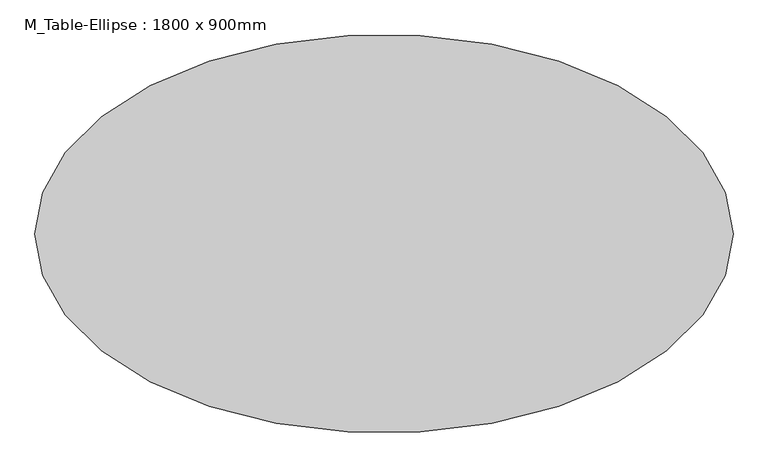
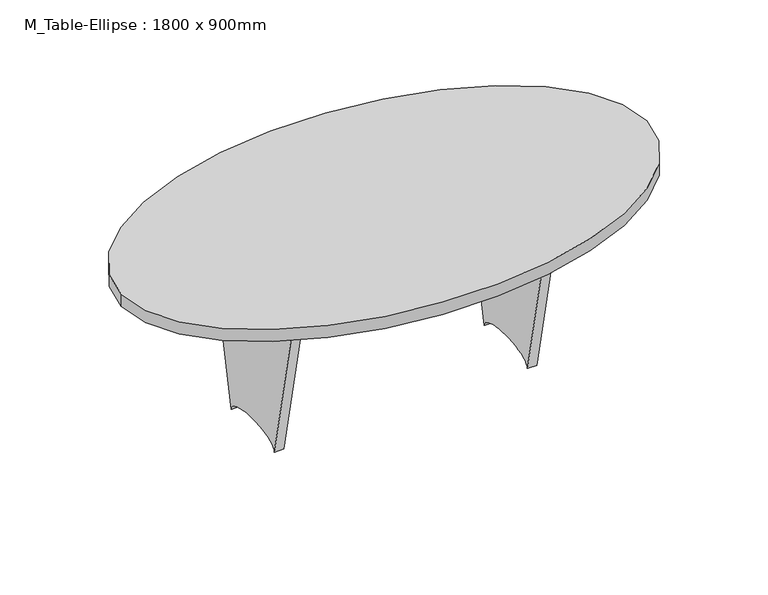
"""IFC4 building model written with IfcOpenShell, lengths in millimetres: furniture geometry, M_Table-Ellipse : 1800 x 900mm."""

from ifc_helpers import new_model, si_unit, point, frame, origin, place, context, project, spatial, ellipse_curve, trimmed, source, transform, mapped, element, save
from ifc_brep_helpers import plane_surface, extruded_surface, advanced_brep


def m_table_ellipse_1800_x_900mm_170b96be(model_context):
    return source(origin(), model_context, "Body", "AdvancedBrep", [
        advanced_brep(
        [(-486.9, 19.05, 709.2), (486.9, 19.05, 709.2), (486.9, 19.05, 472.8), (-486.9, 19.05, 472.8), (-486.9, -19.05, 709.2), (-486.9, -19.05, 472.8), (486.9, -19.05, 472.8), (486.9, -19.05, 709.2)],
        [
            (0, 1),
            (1, 2),
            (2, 3, ellipse_curve(frame((0.0, 19.05, 472.8), z_axis=(0.0, -1.0, 0.0), x_axis=(1.0, 0.0, 0.0)), 486.9, 101.6)),
            (3, 0),
            (4, 5),
            (5, 6, ellipse_curve(frame((0.0, -19.05, 472.8), z_axis=(0.0, 1.0, 0.0), x_axis=(1.0, 0.0, 0.0)), 486.9, 101.6)),
            (6, 7),
            (7, 4),
            (0, 4),
            (7, 1),
            (6, 2),
            (5, 3),
        ],
        [
            plane_surface(frame((-486.9, 19.05, 709.2), z_axis=(0.0, 1.0, 0.0), x_axis=(1.0, 0.0, 0.0))),
            plane_surface(frame((-486.9, -19.05, 709.2), z_axis=(0.0, -1.0, 0.0), x_axis=(-1.0, 0.0, 0.0))),
            plane_surface(frame((-486.9, 19.05, 709.2), z_axis=(0.0, 0.0, 1.0), x_axis=(0.0, -1.0, 0.0))),
            plane_surface(frame((486.9, 19.05, 709.2), z_axis=(1.0, 0.0, 0.0), x_axis=(0.0, -1.0, 0.0))),
            extruded_surface(trimmed(ellipse_curve(frame((0.0, -57.15, 472.8), z_axis=(0.0, -1.0, 0.0), x_axis=(1.0, 0.0, 0.0)), 486.9, 101.6), [point((486.9, -57.15, 472.8))], [point((-486.9, -57.15, 472.8))], True, "CARTESIAN"), (0.0, 38.099999999999994, 0.0), 38.099999999999994),
            plane_surface(frame((-486.9, 19.05, 472.8), z_axis=(-1.0, 0.0, 0.0), x_axis=(0.0, -1.0, 0.0))),
        ],
        [
            (0, [[1, 2, 3, 4]]),
            (1, [[5, 6, 7, 8]]),
            (2, [[-1, 9, -8, 10]]),
            (3, [[-2, -10, -7, 11]]),
            (4, [[-3, -11, -6, 12]]),
            (5, [[-4, -12, -5, -9]]),
        ],
    ),
        advanced_brep(
        [(525.0, 300.0, 709.2), (525.0, -300.0, 709.2), (525.0, -150.0, 0.0), (525.0, 150.0, 0.0), (486.9, 300.0, 709.2), (486.9, 150.0, 0.0), (486.9, -150.0, 0.0), (486.9, -300.0, 709.2)],
        [
            (0, 1),
            (1, 2),
            (2, 3, ellipse_curve(frame((525.0, 0.0, 0.0), z_axis=(-1.0, 0.0, 0.0), x_axis=(0.0, 1.0, 0.0)), 150.0, 50.8)),
            (3, 0),
            (4, 5),
            (5, 6, ellipse_curve(frame((486.9, 0.0, 0.0), z_axis=(1.0, 0.0, 0.0), x_axis=(0.0, 1.0, 0.0)), 150.0, 50.8)),
            (6, 7),
            (7, 4),
            (0, 4),
            (7, 1),
            (6, 2),
            (5, 3),
        ],
        [
            plane_surface(frame((525.0, -300.0, 709.2), z_axis=(1.0, 0.0, 0.0), x_axis=(0.0, -1.0, 0.0))),
            plane_surface(frame((486.9, -300.0, 709.2), z_axis=(-1.0, 0.0, 0.0), x_axis=(0.0, 1.0, 0.0))),
            plane_surface(frame((525.0, 300.0, 709.2), z_axis=(0.0, 0.0, 1.0), x_axis=(-1.0, 0.0, 0.0))),
            plane_surface(frame((525.0, -300.0, 709.2), z_axis=(0.0, -0.9783561485468907, -0.206928119405011), x_axis=(-1.0, 0.0, 0.0))),
            extruded_surface(trimmed(ellipse_curve(frame((448.8, 0.0, 0.0), z_axis=(-1.0, 0.0, 0.0), x_axis=(0.0, 1.0, 0.0)), 150.0, 50.8), [point((448.8, -150.0, 0.0))], [point((448.8, 150.0, 0.0))], True, "CARTESIAN"), (38.099999999999966, 0.0, 0.0), 38.099999999999966),
            plane_surface(frame((525.0, 150.0, 0.0), z_axis=(0.0, 0.9783561485468916, -0.2069281194050069), x_axis=(-1.0, 0.0, 0.0))),
        ],
        [
            (0, [[1, 2, 3, 4]]),
            (1, [[5, 6, 7, 8]]),
            (2, [[-1, 9, -8, 10]]),
            (3, [[-2, -10, -7, 11]]),
            (4, [[-3, -11, -6, 12]]),
            (5, [[-4, -12, -5, -9]]),
        ],
    ),
        advanced_brep(
        [(-486.9, 300.0, 709.2), (-486.9, -300.0, 709.2), (-486.9, -150.0, 0.0), (-486.9, 150.0, 0.0), (-525.0, 300.0, 709.2), (-525.0, 150.0, 0.0), (-525.0, -150.0, 0.0), (-525.0, -300.0, 709.2)],
        [
            (0, 1),
            (1, 2),
            (2, 3, ellipse_curve(frame((-486.9, 0.0, 0.0), z_axis=(-1.0, 0.0, 0.0), x_axis=(0.0, 1.0, 0.0)), 150.0, 50.8)),
            (3, 0),
            (4, 5),
            (5, 6, ellipse_curve(frame((-525.0, 0.0, 0.0), z_axis=(1.0, 0.0, 0.0), x_axis=(0.0, 1.0, 0.0)), 150.0, 50.8)),
            (6, 7),
            (7, 4),
            (0, 4),
            (7, 1),
            (6, 2),
            (5, 3),
        ],
        [
            plane_surface(frame((-486.9, -300.0, 709.2), z_axis=(1.0, 0.0, 0.0), x_axis=(0.0, -1.0, 0.0))),
            plane_surface(frame((-525.0, -300.0, 709.2), z_axis=(-1.0, 0.0, 0.0), x_axis=(0.0, 1.0, 0.0))),
            plane_surface(frame((-486.9, 300.0, 709.2), z_axis=(0.0, 0.0, 1.0), x_axis=(-1.0, 0.0, 0.0))),
            plane_surface(frame((-486.9, -300.0, 709.2), z_axis=(0.0, -0.9783561485468887, -0.2069281194050206), x_axis=(-1.0, 0.0, 0.0))),
            extruded_surface(trimmed(ellipse_curve(frame((-563.1, 0.0, 0.0), z_axis=(-1.0, 0.0, 0.0), x_axis=(0.0, 1.0, 0.0)), 150.0, 50.8), [point((-563.1, -150.0, 0.0))], [point((-563.1, 150.0, 0.0))], True, "CARTESIAN"), (38.10000000000002, 0.0, 0.0), 38.10000000000002),
            plane_surface(frame((-486.9, 150.0, 0.0), z_axis=(0.0, 0.9783561485468906, -0.2069281194050115), x_axis=(-1.0, 0.0, 0.0))),
        ],
        [
            (0, [[1, 2, 3, 4]]),
            (1, [[5, 6, 7, 8]]),
            (2, [[-1, 9, -8, 10]]),
            (3, [[-2, -10, -7, 11]]),
            (4, [[-3, -11, -6, 12]]),
            (5, [[-4, -12, -5, -9]]),
        ],
    ),
        advanced_brep(
        [(-1050.0, 0.0, 760.0), (1050.0, 0.0, 760.0), (-1050.0, 0.0, 709.2), (1050.0, 0.0, 709.2)],
        [
            (0, 1, ellipse_curve(frame((0.0, 0.0, 760.0), z_axis=(0.0, 0.0, 1.0), x_axis=(1.0, 0.0, 0.0)), 1050.0, 600.0)),
            (1, 0, ellipse_curve(frame((0.0, 0.0, 760.0), z_axis=(0.0, 0.0, 1.0), x_axis=(1.0, 0.0, 0.0)), 1050.0, 600.0)),
            (2, 3, ellipse_curve(frame((0.0, 0.0, 709.2), z_axis=(0.0, 0.0, -1.0), x_axis=(1.0, 0.0, 0.0)), 1050.0, 600.0)),
            (3, 2, ellipse_curve(frame((0.0, 0.0, 709.2), z_axis=(0.0, 0.0, -1.0), x_axis=(1.0, 0.0, 0.0)), 1050.0, 600.0)),
            (0, 2),
            (3, 1),
        ],
        [
            plane_surface(frame((1050.0, 0.0, 760.0), z_axis=(0.0, 0.0, 1.0), x_axis=(0.0, 1.0, 0.0))),
            plane_surface(frame((1050.0, 0.0, 709.2), z_axis=(0.0, 0.0, -1.0), x_axis=(0.0, -1.0, 0.0))),
            extruded_surface(trimmed(ellipse_curve(frame((0.0, 0.0, 658.4), z_axis=(0.0, 0.0, 1.0), x_axis=(1.0, 0.0, 0.0)), 1050.0, 600.0), [point((-1050.0, 0.0, 658.4))], [point((1050.0, 0.0, 658.4))], True, "CARTESIAN"), (0.0, 0.0, 50.80000000000007), 50.80000000000007),
            extruded_surface(trimmed(ellipse_curve(frame((0.0, 0.0, 658.4), z_axis=(0.0, 0.0, 1.0), x_axis=(1.0, 0.0, 0.0)), 1050.0, 600.0), [point((1050.0, 0.0, 658.4))], [point((-1050.0, 0.0, 658.4))], True, "CARTESIAN"), (0.0, 0.0, 50.80000000000007), 50.80000000000007),
        ],
        [
            (0, [[1, 2]]),
            (1, [[3, 4]]),
            (2, [[-1, 5, -4, 6]]),
            (3, [[-2, -6, -3, -5]]),
        ],
    ),
    ])


if __name__ == "__main__":
    model = new_model("IFC4")
    model_context = context("Model", 3, world=origin())
    ifc_project = project(units=[si_unit("LENGTHUNIT", "METRE", prefix="MILLI")], contexts=[model_context])
    site = spatial("IfcSite", under=ifc_project)
    building = spatial("IfcBuilding", under=site)
    placement = place(None, origin())
    m_table_ellipse_1800_x_900mm_shape = m_table_ellipse_1800_x_900mm_170b96be(model_context)
    element("IfcFurniture", 1, ObjectType="M_Table-Ellipse : 1800 x 900mm", at=placement, inside=building, context=model_context, shape_type="MappedRepresentation", body=[
        mapped(m_table_ellipse_1800_x_900mm_shape, transform((0.0, 0.0, 0.0), x_axis=(1.0, 0.0, 0.0), y_axis=(0.0, 1.0, 0.0), z_axis=(0.0, 0.0, 1.0))),
    ])
    save(model, "model.ifc")

# Revit data of these elements
# Type "M_Table-Ellipse : 1800 x 900mm"
#   COBie.Type.CreatedBy = "design@eagle.com"
#   COBie.Type.CreatedOn = "2016-09-13T05:47:35"
#   COBie.Type.Name = "Furniture_M_Table-Ellipse_1800 x 900mm"
#   COBie.Type.Category = "23-40 70 14 64 11 : Office Furniture"
#   COBie.Type.Description = ""
#   COBie.Type.Manufacturer = ""
#   COBie.Type.ModelNumber = ""
#   COBie.Type.ReplacementCost = 0
#   Half Width = 600 mm
#   Half Length = 1050 mm
#   Height = 760 mm
#   Length = 2100 mm
#   Width = 1200 mm
#   COBie.Type = yes
#   Base Material = Birch
#   Top Material = Laminate - Black
#   Assembly Code = ""
# Element 1 (IfcFurniture, "M_Table-Ellipse : 1800 x 900mm")
#   Materials on its faces: "Birch", "Laminate - Black"
# Materials
#   "Birch": class "Wood", colour RGB 224 178 126, transparency 0, Description = "Betula Alleghaniensis", Cost = 0
#   "Laminate - Black": class "Miscellaneous", colour RGB 0 0 0, transparency 0
